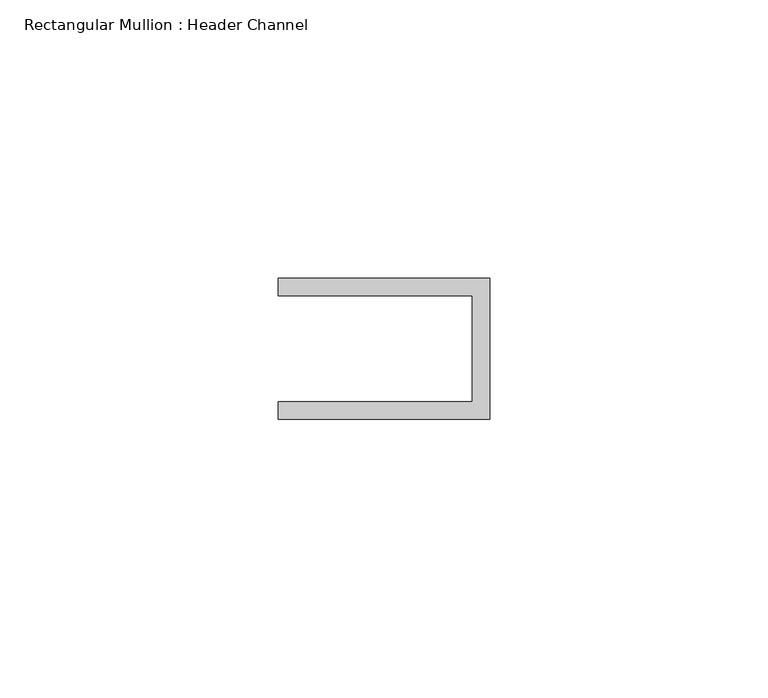
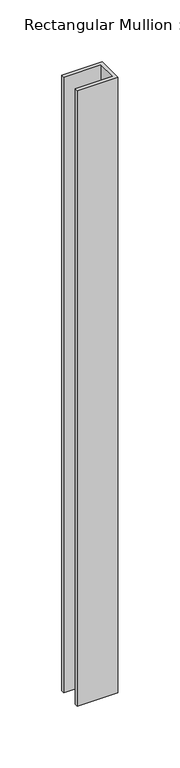
"""IFC4 building model written with IfcOpenShell, lengths in millimetres: member geometry, Rectangular Mullion : Header Channel."""

from ifc_helpers import new_model, si_unit, frame, origin, place, context, project, spatial, polyline, outline, extrude, source, transform, mapped, element, save


def rectangular_mullion_header_channel_c561dbbf(model_context):
    return source(origin(), model_context, "Body", "SweptSolid", [
        extrude(outline(polyline([(0.0, 12.7), (0.0, -12.7), (-38.1, -12.7), (-38.1, -9.525), (-3.175, -9.525), (-3.175, 9.525), (-38.1, 9.525), (-38.1, 12.7), (0.0, 12.7)])), frame((0.0, 0.0, -609.6), z_axis=(0.0, 0.0, 1.0), x_axis=(1.0, 0.0, 0.0)), (0.0, 0.0, 1.0), 609.6),
    ])


if __name__ == "__main__":
    model = new_model("IFC4")
    model_context = context("Model", 3, world=origin())
    ifc_project = project(units=[si_unit("LENGTHUNIT", "METRE", prefix="MILLI")], contexts=[model_context])
    site = spatial("IfcSite", under=ifc_project)
    building = spatial("IfcBuilding", under=site)
    placement = place(None, origin())
    rectangular_mullion_header_channel_shape = rectangular_mullion_header_channel_c561dbbf(model_context)
    element("IfcMember", 1, ObjectType="Rectangular Mullion : Header Channel", at=placement, inside=building, context=model_context, shape_type="MappedRepresentation", body=[
        mapped(rectangular_mullion_header_channel_shape, transform((0.0, 0.0, 0.0), x_axis=(1.0, 0.0, 0.0), y_axis=(0.0, 1.0, 0.0), z_axis=(0.0, 0.0, 1.0))),
    ])
    save(model, "model.ifc")

# Revit data of these elements
# Type "Rectangular Mullion : Header Channel"
#   built-in parameter 1007322 = 0.0833333 (stored number, unit not read)
#   built-in parameter 1007321 = -0.03125 (stored number, unit not read)
#   built-in parameter 1007320 = 0.0416667 (stored number, unit not read)
# Element 1 (IfcMember, "Rectangular Mullion : Header Channel")
#   Materials on its faces: "ALUM"
# Materials
#   "ALUM": class "Generic", colour RGB 157 157 157, transparency 0, Cost = 0
